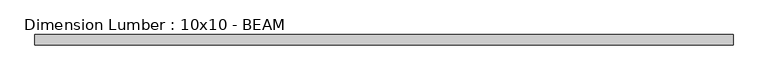
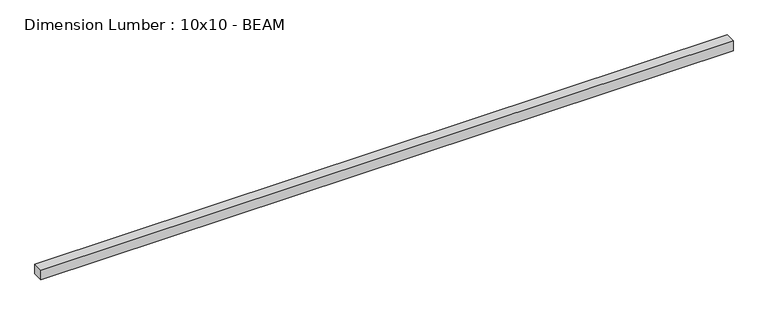
"""IFC4 building model written with IfcOpenShell, lengths in millimetres: beam geometry, Dimension Lumber : 10x10 - BEAM."""

import ifcopenshell
import ifcopenshell.guid

model = None  # the IFC model being written
_history = None  # IfcOwnerHistory: only IFC2X3 demands one
_inside = {}  # id of a spatial element -> (the spatial element, [elements in it])
_under = {}  # id of a project, library or spatial element -> (it, [spatial elements below it])
_declared = {}  # id of a project -> (the project, [libraries it declares])
_typed = {}  # id of a type object -> (the type object, [elements of that type])
_made_of = {}  # id of a material, layer set ... -> (it, [elements and type objects made of it])


def new_model(schema):
    """Start an empty IFC model of exactly this schema.

    Asked for "IFC4X3", IfcOpenShell would pick the latest addendum, in which some entities
    have other attributes; the version numbers below select the first issue.
    IFC2X3 requires an IfcOwnerHistory on every rooted entity: one is made here for all.
    """
    global model, _history
    if schema == "IFC4X3":
        model = ifcopenshell.file(schema_version=(4, 3, 0, 0))
    else:
        model = ifcopenshell.file(schema=schema)
    _inside.clear()
    _under.clear()
    _declared.clear()
    _typed.clear()
    _made_of.clear()
    _history = None
    if model.schema == "IFC2X3":
        org = make("IfcOrganization", Name="unknown")
        user = make(
            "IfcPersonAndOrganization",
            ThePerson=make("IfcPerson", FamilyName="unknown"),
            TheOrganization=org,
        )
        app = make(
            "IfcApplication",
            ApplicationDeveloper=org,
            Version="unknown",
            ApplicationFullName="unknown",
            ApplicationIdentifier="unknown",
        )
        _history = make(
            "IfcOwnerHistory",
            OwningUser=user,
            OwningApplication=app,
            ChangeAction="ADDED",
            CreationDate=0,
        )
    return model


def make(cls, **values):
    """One entity of the class cls with the attributes given. An attribute that is None is left unset."""
    return model.create_entity(
        cls, **{name: value for name, value in values.items() if value is not None}
    )


def rooted(cls, **values):
    """An entity with a GlobalId (a new one), such as an element, a storey or a relation."""
    return make(cls, GlobalId=ifcopenshell.guid.new(), OwnerHistory=_history, **values)


def si_unit(unit_type, name, prefix=None):
    """IfcSIUnit, for example si_unit("LENGTHUNIT", "METRE", prefix="MILLI")."""
    return make("IfcSIUnit", UnitType=unit_type, Prefix=prefix, Name=name)


def assignment(units):
    """IfcUnitAssignment: the units of a project."""
    return None if units is None else make("IfcUnitAssignment", Units=units)


def point(xyz):
    """IfcCartesianPoint."""
    return None if xyz is None else make("IfcCartesianPoint", Coordinates=xyz)


def direction(xyz):
    """IfcDirection."""
    return None if xyz is None else make("IfcDirection", DirectionRatios=xyz)


def frame(location, z_axis=None, x_axis=None):
    """IfcAxis2Placement3D, a coordinate frame: its origin and axes. An axis left out is left unset."""
    return make(
        "IfcAxis2Placement3D",
        Location=point(location),
        Axis=direction(z_axis),
        RefDirection=direction(x_axis),
    )


def origin():
    """The frame at (0, 0, 0) with its axes left unset."""
    return frame((0.0, 0.0, 0.0))


def place(relative_to, where):
    """IfcLocalPlacement: puts the frame where relative to a parent placement (None: the world)."""
    return make(
        "IfcLocalPlacement", PlacementRelTo=relative_to, RelativePlacement=where
    )


def context(
    kind, dimensions, precision=None, world=None, true_north=None, identifier=None
):
    """IfcGeometricRepresentationContext, for example the 3D "Model" context."""
    return make(
        "IfcGeometricRepresentationContext",
        ContextIdentifier=identifier,
        ContextType=kind,
        CoordinateSpaceDimension=dimensions,
        Precision=precision,
        WorldCoordinateSystem=world,
        TrueNorth=true_north,
    )


def project(units=None, contexts=None):
    """IfcProject with its units and contexts."""
    return rooted(
        "IfcProject",
        Name="project",
        RepresentationContexts=contexts,
        UnitsInContext=assignment(units),
    )


def spatial(cls, under=None, at=None, **own):
    """A site, building, storey or space (cls), placed at a placement, below another one or the project."""
    s = rooted(cls, ObjectPlacement=at, **own)
    if under is not None:
        _under.setdefault(under.id(), (under, []))[1].append(s)
    return s


def polyline(points):
    """IfcPolyline through the points."""
    return make("IfcPolyline", Points=[point(p) for p in points])


def outline(outer, holes=None, kind="AREA"):
    """IfcArbitraryClosedProfileDef: a profile drawn as a closed curve; with holes, ...WithVoids."""
    if holes is None:
        return make("IfcArbitraryClosedProfileDef", ProfileType=kind, OuterCurve=outer)
    return make(
        "IfcArbitraryProfileDefWithVoids",
        ProfileType=kind,
        OuterCurve=outer,
        InnerCurves=holes,
    )


def extrude(swept, where, along, depth):
    """IfcExtrudedAreaSolid: the profile swept, set in the frame where, extruded along a direction by depth."""
    return make(
        "IfcExtrudedAreaSolid",
        SweptArea=swept,
        Position=where,
        ExtrudedDirection=direction(along),
        Depth=depth,
    )


def shape(context_of_items, identifier, shape_type, items):
    """IfcShapeRepresentation: the items that make up one representation, for example the "Body"."""
    return make(
        "IfcShapeRepresentation",
        ContextOfItems=context_of_items,
        RepresentationIdentifier=identifier,
        RepresentationType=shape_type,
        Items=items,
    )


def source(mapping_origin, context_of_items, identifier, shape_type, items):
    """IfcRepresentationMap: a shape defined once, which mapped items show again and again."""
    return make(
        "IfcRepresentationMap",
        MappingOrigin=mapping_origin,
        MappedRepresentation=shape(context_of_items, identifier, shape_type, items),
    )


def transform(
    local_origin,
    x_axis=None,
    y_axis=None,
    z_axis=None,
    scale=None,
    scale2=None,
    scale3=None,
    uniform=True,
):
    """IfcCartesianTransformationOperator3D, or its non-uniform kind. x_axis, y_axis, z_axis: its Axis1, 2, 3."""
    if uniform:
        return make(
            "IfcCartesianTransformationOperator3D",
            Axis1=direction(x_axis),
            Axis2=direction(y_axis),
            LocalOrigin=point(local_origin),
            Scale=scale,
            Axis3=direction(z_axis),
        )
    return make(
        "IfcCartesianTransformationOperator3DnonUniform",
        Axis1=direction(x_axis),
        Axis2=direction(y_axis),
        LocalOrigin=point(local_origin),
        Scale=scale,
        Axis3=direction(z_axis),
        Scale2=scale2,
        Scale3=scale3,
    )


def mapped(mapping_source, mapping_target):
    """IfcMappedItem: shows the shape of a source again, moved by a transform."""
    return make(
        "IfcMappedItem", MappingSource=mapping_source, MappingTarget=mapping_target
    )


def made_of(thing, what):
    """Note that an element or type object is made of a material, layer set ...; save() writes the relation."""
    if what is not None:
        _made_of.setdefault(what.id(), (what, []))[1].append(thing)
    return thing


def element(
    cls,
    number,
    at=None,
    inside=None,
    cuts=None,
    type_object=None,
    material=None,
    context=None,
    identifier="Body",
    shape_type=None,
    held_by="IfcProductDefinitionShape",
    body=None,
    shapes=None,
    **own,
):
    """One element of the class cls, such as IfcWall. Its Tag is "e" and its number.

    at: its placement. inside: the storey or other place that contains it. cuts: it is an
    opening in that element (IfcRelVoidsElement). A single representation is given by context,
    identifier, shape_type and body (its items); several are given by shapes. held_by: the class
    of the entity that holds the representations. save() writes the other relations.
    """
    e = rooted(cls, Tag="e%d" % number, ObjectPlacement=at, **own)
    if body is not None:
        shapes = [shape(context, identifier, shape_type, body)]
    if shapes is not None:
        e.Representation = make(held_by, Representations=shapes)
    if inside is not None:
        _inside.setdefault(inside.id(), (inside, []))[1].append(e)
    if cuts is not None:
        rooted(
            "IfcRelVoidsElement", RelatingBuildingElement=cuts, RelatedOpeningElement=e
        )
    if type_object is not None:
        _typed.setdefault(type_object.id(), (type_object, []))[1].append(e)
    return made_of(e, material)


def aggregate(whole, parts):
    """IfcRelAggregates: a whole, such as a stair, and the parts it consists of."""
    return rooted("IfcRelAggregates", RelatingObject=whole, RelatedObjects=parts)


def save(model, path):
    """Write the relations noted so far, then the file.

    IfcRelAggregates (storeys below a building ...), IfcRelContainedInSpatialStructure (elements
    in a storey), IfcRelDefinesByType, IfcRelAssociatesMaterial and IfcRelDeclares: one each for
    every whole, place, type object, material and project.
    """
    for whole, parts in _under.values():
        aggregate(whole, parts)
    for where, things in _inside.values():
        rooted(
            "IfcRelContainedInSpatialStructure",
            RelatedElements=things,
            RelatingStructure=where,
        )
    for kind, things in _typed.values():
        rooted("IfcRelDefinesByType", RelatedObjects=things, RelatingType=kind)
    for what, things in _made_of.values():
        rooted("IfcRelAssociatesMaterial", RelatedObjects=things, RelatingMaterial=what)
    for by, libraries in _declared.values():
        rooted("IfcRelDeclares", RelatingContext=by, RelatedDefinitions=libraries)
    model.write(path)


def dimension_lumber_10x10_beam_babce44f(model_context):
    return source(origin(), model_context, "Body", "SweptSolid", [
        extrude(outline(polyline([(7924.8, 117.475), (7924.8, -117.475), (-7924.8, -117.475), (-7924.8, 117.475), (7924.8, 117.475)])), frame((0.0, 0.0, -117.475), z_axis=(0.0, 0.0, 1.0), x_axis=(1.0, 0.0, 0.0)), (0.0, 0.0, 1.0), 234.95),
    ])


if __name__ == "__main__":
    model = new_model("IFC4")
    model_context = context("Model", 3, world=origin())
    ifc_project = project(units=[si_unit("LENGTHUNIT", "METRE", prefix="MILLI")], contexts=[model_context])
    site = spatial("IfcSite", under=ifc_project)
    building = spatial("IfcBuilding", under=site)
    placement = place(None, origin())
    dimension_lumber_10x10_beam_shape = dimension_lumber_10x10_beam_babce44f(model_context)
    element("IfcBeam", 1, ObjectType="Dimension Lumber : 10x10 - BEAM", at=placement, inside=building, context=model_context, shape_type="MappedRepresentation", body=[
        mapped(dimension_lumber_10x10_beam_shape, transform((0.0, 0.0, 0.0), x_axis=(1.0, 0.0, 0.0), y_axis=(0.0, 1.0, 0.0), z_axis=(0.0, 0.0, 1.0))),
    ])
    save(model, "model.ifc")

# Revit data of these elements
# Type "Dimension Lumber : 10x10 - BEAM"
#   Assembly Code = "B10"
#   A = 0.0755556 SF
#   Length [instance default] = 5' - 0"
#   b = 0' - 9 1/4"
#   d = 0' - 9 1/4"
#   Structural Material = (4) CHARRED SISTERED 2X10s AT BEAM
# Element 1 (IfcBeam, "Dimension Lumber : 10x10 - BEAM")
#   Materials on its faces: "(4) CHARRED SISTERED 2X10s AT BEAM"
# Materials
#   "(4) CHARRED SISTERED 2X10s AT BEAM": class "Wood", colour RGB 144 144 144, transparency 0, Description = "Pinus Echinata", Cost = 0
